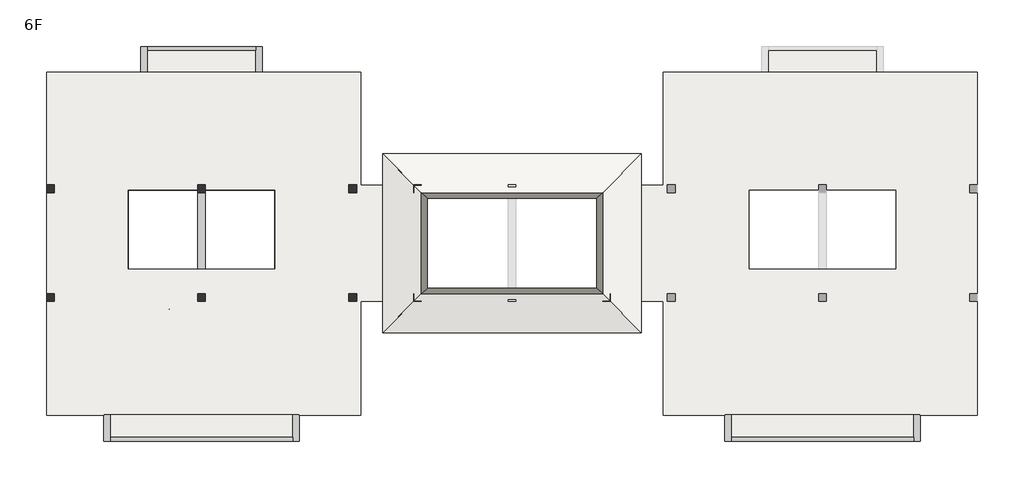
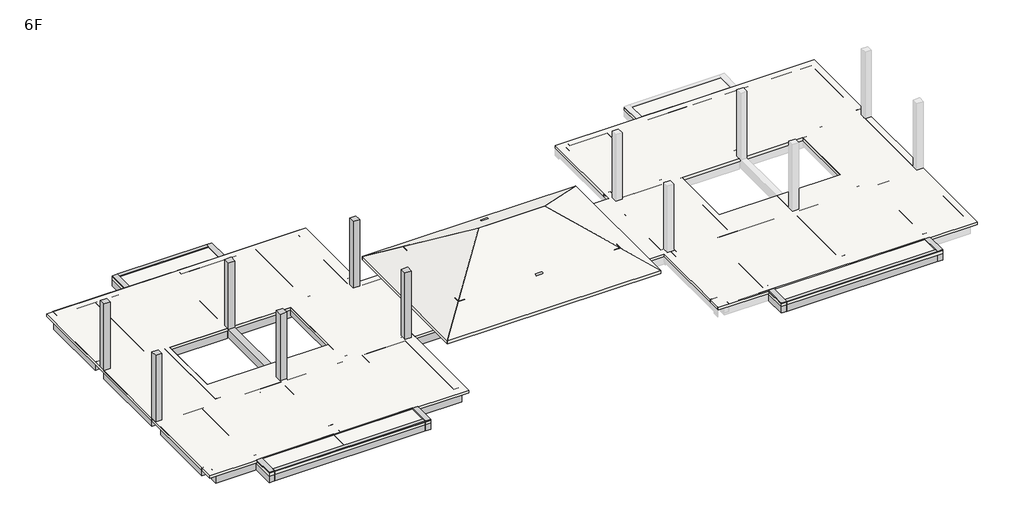
# One storey, part 1 of 2: 38 beams, 8 columns, 6 slabs.
"""IFC4 building model written with IfcOpenShell, lengths in millimetres."""

from ifc_helpers import new_model, si_unit, frame, origin, place, context, project, spatial, polyline, outline, extrude, faceted_brep, element, save

model = new_model("IFC4")

# Units and contexts
model_context = context("Model", 3, world=origin())
ifc_project = project(units=[si_unit("LENGTHUNIT", "METRE", prefix="MILLI")], contexts=[model_context])

# Site, building, storey
site = spatial("IfcSite", under=ifc_project)
building = spatial("IfcBuilding", under=site)
storey = spatial("IfcBuildingStorey", under=building, Name="6F", Elevation=17230.0)

# Beams
placement = place(None, origin())
element("IfcBeam", 1, ObjectType="M_Concrete-Rectangular Beam : 150x500", at=placement, inside=storey, context=model_context, shape_type="SweptSolid", body=[
    extrude(outline(polyline([(2320.0000398, -1149.9999999), (2320.0000398, -999.9999999), (9380.0000399, -999.9999999), (9380.0000399, -1149.9999999), (2320.0000398, -1149.9999999)])), frame((0.0, 0.0, 16730.0), z_axis=(0.0, 0.0, 1.0), x_axis=(1.0, 0.0, 0.0)), (0.0, 0.0, 1.0), 500.0),
])
element("IfcBeam", 2, ObjectType="M_Concrete-Rectangular Beam : 150x500", at=placement, inside=storey, context=model_context, shape_type="SweptSolid", body=[
    extrude(outline(polyline([(26320.012858, -1149.9999998), (26320.012858, -999.9999998), (33380.0128581, -999.9999998), (33380.0128581, -1149.9999998), (26320.012858, -1149.9999998)])), frame((0.0, 0.0, 16730.0), z_axis=(0.0, 0.0, 1.0), x_axis=(1.0, 0.0, 0.0)), (0.0, 0.0, 1.0), 500.0),
])
element("IfcBeam", 3, ObjectType="M_Concrete-Rectangular Beam : 150x500", at=placement, inside=storey, context=model_context, shape_type="SweptSolid", body=[
    extrude(outline(polyline([(7940.0998269, 14100.0000002), (7940.0998269, 13950.0000002), (3759.9001745, 13950.0000002), (3759.9001745, 14100.0000002), (7940.0998269, 14100.0000002)])), frame((0.0, 0.0, 16730.0), z_axis=(0.0, 0.0, 1.0), x_axis=(1.0, 0.0, 0.0)), (0.0, 0.0, 1.0), 500.0),
])
element("IfcBeam", 4, ObjectType="M_Concrete-Rectangular Beam : 250x400", at=placement, inside=storey, context=model_context, shape_type="Brep", body=[
    faceted_brep([(8930.0, 8549.9999993, 17230.0), (8680.0, 8549.9999993, 17230.0), (8680.0, 4449.9999998, 17230.0), (8930.0, 4449.9999998, 17230.0), (8680.0, 8549.9999993, 17088.8582236), (8680.0, 8549.9999993, 16830.0), (8680.0, 4449.9999998, 16830.0), (8930.0, 8549.9999993, 16830.0), (8930.0, 4449.9999998, 16830.0)], [[[0, 1, 2, 3]], [[1, 4, 5, 6, 2]], [[5, 7, 8, 6]], [[7, 0, 3, 8]], [[1, 0, 7, 5, 4]], [[3, 2, 6, 8]]]),
])
element("IfcBeam", 5, ObjectType="M_Concrete-Rectangular Beam : 250x400", at=placement, inside=storey, context=model_context, shape_type="SweptSolid", body=[
    extrude(outline(polyline([(14050.0174941, 8449.9999993), (14300.0174941, 8449.9999993), (14300.0174941, 4549.9999902), (14050.0174941, 4549.9999902), (14050.0174941, 8449.9999993)])), frame((0.0, 0.0, 16830.0), z_axis=(0.0, 0.0, 1.0), x_axis=(1.0, 0.0, 0.0)), (0.0, 0.0, 1.0), 400.0),
])
element("IfcBeam", 6, ObjectType="M_Concrete-Rectangular Beam : 250x400", at=placement, inside=storey, context=model_context, shape_type="Brep", body=[
    faceted_brep([(3020.0, 8549.9999993, 17230.0), (2770.0, 8549.9999993, 17230.0), (2770.0, 4449.9999998, 17230.0), (3020.0, 4449.9999998, 17230.0), (3020.0, 8549.9999993, 16830.0), (3020.0, 8549.9999993, 17088.8582245), (3020.0, 4449.9999998, 16830.0), (2770.0, 8549.9999993, 16830.0), (2770.0, 4449.9999998, 16830.0)], [[[0, 1, 2, 3]], [[4, 5, 0, 3, 6]], [[7, 4, 6, 8]], [[1, 7, 8, 2]], [[1, 0, 5, 4, 7]], [[3, 2, 8, 6]]]),
])
element("IfcBeam", 7, ObjectType="M_Concrete-Rectangular Beam : 250x400", at=placement, inside=storey, context=model_context, shape_type="SweptSolid", body=[
    extrude(outline(polyline([(1965.3131971, 12800.0000001), (2215.3131971, 12800.0000001), (2215.3131971, 8849.9999993), (1965.3131971, 8849.9999993), (1965.3131971, 12800.0000001)])), frame((0.0, 0.0, 16830.0), z_axis=(0.0, 0.0, 1.0), x_axis=(1.0, 0.0, 0.0)), (0.0, 0.0, 1.0), 400.0),
])
element("IfcBeam", 8, ObjectType="M_Concrete-Rectangular Beam : 250x400", at=placement, inside=storey, context=model_context, shape_type="SweptSolid", body=[
    extrude(outline(polyline([(1965.3131971, 4149.9999998), (2215.3131971, 4149.9999998), (2215.3131971, 199.9999993), (1965.3131971, 199.9999993), (1965.3131971, 4149.9999998)])), frame((0.0, 0.0, 16830.0), z_axis=(0.0, 0.0, 1.0), x_axis=(1.0, 0.0, 0.0)), (0.0, 0.0, 1.0), 400.0),
])
element("IfcBeam", 9, ObjectType="M_Concrete-Rectangular Beam : 250x400", at=placement, inside=storey, context=model_context, shape_type="SweptSolid", body=[
    extrude(outline(polyline([(9485.2332382, 12800.0000001), (9735.2332382, 12800.0000001), (9735.2332382, 8849.9999993), (9485.2332382, 8849.9999993), (9485.2332382, 12800.0000001)])), frame((0.0, 0.0, 16830.0), z_axis=(0.0, 0.0, 1.0), x_axis=(1.0, 0.0, 0.0)), (0.0, 0.0, 1.0), 400.0),
])
element("IfcBeam", 10, ObjectType="M_Concrete-Rectangular Beam : 250x400", at=placement, inside=storey, context=model_context, shape_type="SweptSolid", body=[
    extrude(outline(polyline([(9485.2332382, 4149.9999998), (9735.2332382, 4149.9999998), (9735.2332382, 199.9999993), (9485.2332382, 199.9999993), (9485.2332382, 4149.9999998)])), frame((0.0, 0.0, 16830.0), z_axis=(0.0, 0.0, 1.0), x_axis=(1.0, 0.0, 0.0)), (0.0, 0.0, 1.0), 400.0),
])
element("IfcBeam", 11, ObjectType="M_Concrete-Rectangular Beam : 250x400", at=placement, inside=storey, context=model_context, shape_type="SweptSolid", body=[
    extrude(outline(polyline([(17780.0, 14075.0174936), (17780.0, 14325.0174936), (18180.0, 14325.0174936), (18180.0, 14191.5713263), (18102.3013889, 14075.0174936), (17780.0, 14075.0174936)])), frame((0.0, 4550.0000005, 0.0), z_axis=(0.0, 1.0, 0.0), x_axis=(0.0, 0.0, 1.0)), (0.0, 0.0, 1.0), 3899.9999997),
])
element("IfcBeam", 12, ObjectType="M_Concrete-Rectangular Beam : 250x500", at=placement, inside=storey, context=model_context, shape_type="Brep", body=[
    faceted_brep([(3509.9001745, 13101.5853605, 17230.0), (3509.9001745, 13101.5853605, 16730.0), (3759.9001745, 13101.5853605, 16730.0), (3759.9001745, 13101.5853605, 17230.0), (3759.9001745, 13950.0000002, 17230.0), (3759.9001745, 14100.0000002, 17230.0), (3509.9001745, 14100.0000002, 17230.0), (3759.9001745, 13950.0000002, 16730.0), (3759.9001745, 14100.0000002, 16730.0), (3509.9001745, 14100.0000002, 16730.0)], [[[0, 1, 2, 3]], [[0, 3, 4, 5, 6]], [[3, 2, 7, 8, 5, 4]], [[2, 1, 9, 8, 7]], [[1, 0, 6, 9]], [[6, 5, 8, 9]]]),
])
element("IfcBeam", 13, ObjectType="M_Concrete-Rectangular Beam : 250x500", at=placement, inside=storey, context=model_context, shape_type="Brep", body=[
    faceted_brep([(2070.0000398, -1149.9999999, 17230.0), (2320.0000398, -1149.9999999, 17230.0), (2320.0000398, -999.9999999, 17230.0), (2320.0000398, -100.0000007, 17230.0), (2070.0000398, -100.0000007, 17230.0), (2320.0000398, -1149.9999999, 16730.0), (2320.0000398, -999.9999999, 16730.0), (2320.0000398, -100.0000007, 16730.0), (2070.0000398, -1149.9999999, 16730.0), (2070.0000398, -100.0000007, 16730.0)], [[[0, 1, 2, 3, 4]], [[1, 5, 6, 7, 3, 2]], [[5, 8, 9, 7, 6]], [[8, 0, 4, 9]], [[4, 3, 7, 9]], [[1, 0, 8, 5]]]),
])
element("IfcBeam", 14, ObjectType="M_Concrete-Rectangular Beam : 250x500", at=placement, inside=storey, context=model_context, shape_type="Brep", body=[
    faceted_brep([(9380.0000399, -1149.9999999, 17230.0), (9630.0000399, -1149.9999999, 17230.0), (9630.0000399, -100.0000007, 17230.0), (9380.0000399, -100.0000007, 17230.0), (9380.0000399, -999.9999999, 17230.0), (9380.0000399, -1149.9999999, 16730.0), (9380.0000399, -100.0000007, 16730.0), (9380.0000399, -999.9999999, 16730.0), (9630.0000399, -1149.9999999, 16730.0), (9630.0000399, -100.0000007, 16730.0)], [[[0, 1, 2, 3, 4]], [[5, 0, 4, 3, 6, 7]], [[8, 5, 7, 6, 9]], [[1, 8, 9, 2]], [[1, 0, 5, 8]], [[3, 2, 9, 6]]]),
])
element("IfcBeam", 15, ObjectType="M_Concrete-Rectangular Beam : 250x500", at=placement, inside=storey, context=model_context, shape_type="Brep", body=[
    faceted_brep([(26070.012858, -1149.9999998, 17230.0), (26320.012858, -1149.9999998, 17230.0), (26320.012858, -999.9999998, 17230.0), (26320.012858, -100.0000013, 17230.0), (26070.012858, -100.0000013, 17230.0), (26320.012858, -1149.9999998, 16730.0), (26320.012858, -999.9999998, 16730.0), (26320.012858, -100.0000013, 16730.0), (26070.012858, -1149.9999998, 16730.0), (26070.012858, -100.0000013, 16730.0)], [[[0, 1, 2, 3, 4]], [[1, 5, 6, 7, 3, 2]], [[5, 8, 9, 7, 6]], [[8, 0, 4, 9]], [[1, 0, 8, 5]], [[4, 3, 7, 9]]]),
])
element("IfcBeam", 16, ObjectType="M_Concrete-Rectangular Beam : 250x500", at=placement, inside=storey, context=model_context, shape_type="Brep", body=[
    faceted_brep([(33380.0128581, -1149.9999998, 17230.0), (33630.0128581, -1149.9999998, 17230.0), (33630.0128581, -100.0000013, 17230.0), (33380.0128581, -100.0000013, 17230.0), (33380.0128581, -999.9999998, 17230.0), (33380.0128581, -1149.9999998, 16730.0), (33380.0128581, -100.0000013, 16730.0), (33380.0128581, -999.9999998, 16730.0), (33630.0128581, -1149.9999998, 16730.0), (33630.0128581, -100.0000013, 16730.0)], [[[0, 1, 2, 3, 4]], [[5, 0, 4, 3, 6, 7]], [[8, 5, 7, 6, 9]], [[1, 8, 9, 2]], [[1, 0, 5, 8]], [[3, 2, 9, 6]]]),
])
element("IfcBeam", 17, ObjectType="M_Concrete-Rectangular Beam : 250x500", at=placement, inside=storey, context=model_context, shape_type="Brep", body=[
    faceted_brep([(8190.0998269, 14100.0000002, 17230.0), (7940.0998269, 14100.0000002, 17230.0), (7940.0998269, 13950.0000002, 17230.0), (7940.0998269, 13100.0000001, 17230.0), (8190.0998269, 13100.0000001, 17230.0), (8190.0998269, 14100.0000002, 16730.0), (8190.0998269, 13100.0000001, 16730.0), (7940.0998269, 14100.0000002, 16730.0), (7940.0998269, 13100.0000001, 16730.0), (7940.0998269, 13950.0000002, 16730.0)], [[[0, 1, 2, 3, 4]], [[5, 0, 4, 6]], [[7, 5, 6, 8, 9]], [[1, 7, 9, 8, 3, 2]], [[1, 0, 5, 7]], [[4, 3, 8, 6]]]),
])
element("IfcBeam", 18, ObjectType="M_Concrete-Rectangular Beam : 300x400", at=placement, inside=storey, context=model_context, shape_type="SweptSolid", body=[
    extrude(outline(polyline([(165.0, 9150.0000002), (-135.0, 9150.0000002), (-135.0, 12500.0000005), (165.0, 12500.0000005), (165.0, 9150.0000002)])), frame((0.0, 0.0, 16830.0), z_axis=(0.0, 0.0, 1.0), x_axis=(1.0, 0.0, 0.0)), (0.0, 0.0, 1.0), 400.0),
])
element("IfcBeam", 19, ObjectType="M_Concrete-Rectangular Beam : 300x400", at=placement, inside=storey, context=model_context, shape_type="SweptSolid", body=[
    extrude(outline(polyline([(165.0, 4550.0000002), (-135.0, 4550.0000002), (-135.0, 8450.0000002), (165.0, 8450.0000002), (165.0, 4550.0000002)])), frame((0.0, 0.0, 16830.0), z_axis=(0.0, 0.0, 1.0), x_axis=(1.0, 0.0, 0.0)), (0.0, 0.0, 1.0), 400.0),
])
element("IfcBeam", 20, ObjectType="M_Concrete-Rectangular Beam : 300x400", at=placement, inside=storey, context=model_context, shape_type="SweptSolid", body=[
    extrude(outline(polyline([(165.0, 500.0), (-135.0, 500.0), (-135.0, 3850.0000002), (165.0, 3850.0000002), (165.0, 500.0)])), frame((0.0, 0.0, 16830.0), z_axis=(0.0, 0.0, 1.0), x_axis=(1.0, 0.0, 0.0)), (0.0, 0.0, 1.0), 400.0),
])
element("IfcBeam", 21, ObjectType="M_Concrete-Rectangular Beam : 300x400", at=placement, inside=storey, context=model_context, shape_type="SweptSolid", body=[
    extrude(outline(polyline([(6000.0, 4550.0000002), (5700.0, 4550.0000002), (5700.0, 8450.0000002), (6000.0, 8450.0000002), (6000.0, 4550.0000002)])), frame((0.0, 0.0, 16830.0), z_axis=(0.0, 0.0, 1.0), x_axis=(1.0, 0.0, 0.0)), (0.0, 0.0, 1.0), 400.0),
])
element("IfcBeam", 22, ObjectType="M_Concrete-Rectangular Beam : 300x400", at=placement, inside=storey, context=model_context, shape_type="SweptSolid", body=[
    extrude(outline(polyline([(6000.0000007, 500.0), (5700.0000007, 500.0), (5700.0000007, 3850.0000002), (6000.0000007, 3850.0000002), (6000.0000007, 500.0)])), frame((0.0, 0.0, 16830.0), z_axis=(0.0, 0.0, 1.0), x_axis=(1.0, 0.0, 0.0)), (0.0, 0.0, 1.0), 400.0),
])
element("IfcBeam", 23, ObjectType="M_Concrete-Rectangular Beam : 300x400", at=placement, inside=storey, context=model_context, shape_type="SweptSolid", body=[
    extrude(outline(polyline([(6000.0000007, 9150.0000002), (5700.0000007, 9150.0000002), (5700.0000007, 12500.0000005), (6000.0000007, 12500.0000005), (6000.0000007, 9150.0000002)])), frame((0.0, 0.0, 16830.0), z_axis=(0.0, 0.0, 1.0), x_axis=(1.0, 0.0, 0.0)), (0.0, 0.0, 1.0), 400.0),
])
element("IfcBeam", 24, ObjectType="M_Concrete-Rectangular Beam : 300x400", at=placement, inside=storey, context=model_context, shape_type="Brep", body=[
    faceted_brep([(6000.0000007, -100.0, 17180.0), (5700.0000007, -100.0000007, 17180.0), (5700.0000007, -999.9999999, 17180.0), (6000.0000007, -999.9999999, 17180.0), (6000.0000007, -999.9999999, 16780.0), (6000.0000007, -100.0, 16780.0), (5700.0000007, -100.0000007, 16780.0), (5700.0000007, -999.9999999, 16780.0)], [[[0, 1, 2, 3]], [[3, 4, 5, 0]], [[6, 5, 4, 7]], [[1, 6, 7, 2]], [[0, 5, 6, 1]], [[3, 2, 7, 4]]]),
])
element("IfcBeam", 25, ObjectType="M_Concrete-Rectangular Beam : 300x400", at=placement, inside=storey, context=model_context, shape_type="Brep", body=[
    faceted_brep([(30000.0064292, -100.0, 17180.0), (29700.0064292, -100.0000013, 17180.0), (29700.0064292, -999.9999998, 17180.0), (30000.0064292, -999.9999998, 17180.0), (30000.0064292, -999.9999998, 16780.0), (30000.0064292, -100.0, 16780.0), (29700.0064292, -100.0000013, 16780.0), (29700.0064292, -999.9999998, 16780.0)], [[[0, 1, 2, 3]], [[3, 4, 5, 0]], [[6, 5, 4, 7]], [[1, 6, 7, 2]], [[0, 5, 6, 1]], [[3, 2, 7, 4]]]),
])
element("IfcBeam", 26, ObjectType="M_Concrete-Rectangular Beam : 300x500", at=placement, inside=storey, context=model_context, shape_type="Brep", body=[
    faceted_brep([(5700.0000007, 12800.0000001, 17230.0), (5700.0000007, 13100.0000001, 17230.0), (165.0, 13100.0000001, 17230.0), (165.0, 12800.0000001, 17230.0), (1965.3131971, 12800.0000001, 17230.0), (2215.3131971, 12800.0000001, 17230.0), (5700.0000007, 12800.0000001, 16730.0), (165.0, 12800.0000001, 16730.0), (5700.0000007, 13100.0000001, 16730.0), (165.0, 13100.0000001, 16730.0)], [[[0, 1, 2, 3, 4, 5]], [[6, 0, 5, 4, 3, 7]], [[8, 6, 7, 9]], [[1, 8, 9, 2]], [[1, 0, 6, 8]], [[3, 2, 9, 7]]]),
])
element("IfcBeam", 27, ObjectType="M_Concrete-Rectangular Beam : 300x500", at=placement, inside=storey, context=model_context, shape_type="Brep", body=[
    faceted_brep([(164.9649925, 8849.9999993, 17230.0), (164.9649925, 8549.9999993, 17230.0), (2770.0, 8549.9999993, 17230.0), (3020.0, 8549.9999993, 17230.0), (5699.9649933, 8549.9999993, 17230.0), (5699.9649933, 8849.9999993, 17230.0), (2215.3131971, 8849.9999993, 17230.0), (1965.3131971, 8849.9999993, 17230.0), (164.9649925, 8549.9999993, 16730.0), (5699.9649933, 8549.9999993, 16730.0), (164.9649925, 8849.9999993, 16730.0), (5699.9649933, 8849.9999993, 16730.0)], [[[0, 1, 2, 3, 4, 5, 6, 7]], [[1, 8, 9, 4, 3, 2]], [[8, 10, 11, 9]], [[10, 0, 7, 6, 5, 11]], [[1, 0, 10, 8]], [[5, 4, 9, 11]]]),
])
element("IfcBeam", 28, ObjectType="M_Concrete-Rectangular Beam : 300x500", at=placement, inside=storey, context=model_context, shape_type="Brep", body=[
    faceted_brep([(165.0, 4449.9999998, 17230.0), (165.0, 4149.9999998, 17230.0), (1965.3131971, 4149.9999998, 17230.0), (2215.3131971, 4149.9999998, 17230.0), (5700.0000007, 4149.9999998, 17230.0), (5700.0000007, 4449.9999998, 17230.0), (3020.0, 4449.9999998, 17230.0), (2770.0, 4449.9999998, 17230.0), (165.0, 4149.9999998, 16730.0), (5700.0000007, 4149.9999998, 16730.0), (165.0, 4449.9999998, 16730.0), (5700.0000007, 4449.9999998, 16730.0)], [[[0, 1, 2, 3, 4, 5, 6, 7]], [[1, 8, 9, 4, 3, 2]], [[8, 10, 11, 9]], [[10, 0, 7, 6, 5, 11]], [[1, 0, 10, 8]], [[5, 4, 9, 11]]]),
])
element("IfcBeam", 29, ObjectType="M_Concrete-Rectangular Beam : 300x500", at=placement, inside=storey, context=model_context, shape_type="Brep", body=[
    faceted_brep([(165.0, 199.9999993, 17230.0), (165.0, -100.0000007, 17230.0), (2070.0000398, -100.0000007, 17230.0), (2320.0000398, -100.0000007, 17230.0), (5700.0000007, -100.0000007, 17230.0), (5700.0000007, 199.9999993, 17230.0), (2215.3131971, 199.9999993, 17230.0), (1965.3131971, 199.9999993, 17230.0), (165.0, -100.0000007, 16730.0), (2070.0000398, -100.0000007, 16730.0), (2320.0000398, -100.0000007, 16730.0), (5700.0000007, -100.0000007, 16730.0), (165.0, 199.9999993, 16730.0), (5700.0000007, 199.9999993, 16730.0)], [[[0, 1, 2, 3, 4, 5, 6, 7]], [[1, 8, 9, 10, 11, 4, 3, 2]], [[8, 12, 13, 11, 10, 9]], [[12, 0, 7, 6, 5, 13]], [[1, 0, 12, 8]], [[5, 4, 11, 13]]]),
])
element("IfcBeam", 30, ObjectType="M_Concrete-Rectangular Beam : 300x500", at=placement, inside=storey, context=model_context, shape_type="Brep", body=[
    faceted_brep([(6000.0000007, 13100.0000001, 17230.0), (6000.0000007, 12800.0000001, 17230.0), (9485.2332382, 12800.0000001, 17230.0), (9735.2332382, 12800.0000001, 17230.0), (11500.0174948, 12800.0000001, 17230.0), (11700.0000034, 12800.0000001, 17230.0), (11700.0000034, 13100.0000001, 17230.0), (8190.0998269, 13100.0000001, 17230.0), (7940.0998269, 13100.0000001, 17230.0), (6000.0000007, 12800.0000001, 16730.0), (11700.0000034, 12800.0000001, 16730.0), (11700.0000034, 12800.0000001, 16830.0), (6000.0000007, 13100.0000001, 16730.0), (7940.0998269, 13100.0000001, 16730.0), (8190.0998269, 13100.0000001, 16730.0), (11700.0000034, 13100.0000001, 16730.0)], [[[0, 1, 2, 3, 4, 5, 6, 7, 8]], [[1, 9, 10, 11, 5, 4, 3, 2]], [[9, 12, 13, 14, 15, 10]], [[12, 0, 8, 7, 6, 15, 14, 13]], [[1, 0, 12, 9]], [[6, 5, 11, 10, 15]]]),
])
element("IfcBeam", 31, ObjectType="M_Concrete-Rectangular Beam : 300x500", at=placement, inside=storey, context=model_context, shape_type="Brep", body=[
    faceted_brep([(5999.9649933, 8849.9999993, 17230.0), (5999.9649933, 8549.9999993, 17230.0), (8680.0, 8549.9999993, 17230.0), (8930.0, 8549.9999993, 17230.0), (11500.0174941, 8549.9999993, 17230.0), (11699.964996, 8549.9999993, 17230.0), (11699.964996, 8849.9999993, 17230.0), (11500.0174948, 8849.9999993, 17230.0), (9735.2332382, 8849.9999993, 17230.0), (9485.2332382, 8849.9999993, 17230.0), (5999.9649933, 8549.9999993, 16730.0), (11500.0174941, 8549.9999993, 16730.0), (11699.964996, 8549.9999993, 16730.0), (11699.964996, 8549.9999993, 16830.0), (5999.9649933, 8849.9999993, 16730.0), (11699.964996, 8849.9999993, 16730.0), (11699.964996, 8849.9999993, 16830.0)], [[[0, 1, 2, 3, 4, 5, 6, 7, 8, 9]], [[1, 10, 11, 12, 13, 5, 4, 3, 2]], [[10, 14, 15, 12, 11]], [[14, 0, 9, 8, 7, 6, 16, 15]], [[1, 0, 14, 10]], [[6, 5, 13, 12, 15, 16]]]),
])
element("IfcBeam", 32, ObjectType="M_Concrete-Rectangular Beam : 300x500", at=placement, inside=storey, context=model_context, shape_type="Brep", body=[
    faceted_brep([(6000.0000007, 4449.9999998, 17230.0), (6000.0000007, 4149.9999998, 17230.0), (9485.2332382, 4149.9999998, 17230.0), (9735.2332382, 4149.9999998, 17230.0), (11500.0174948, 4149.9999998, 17230.0), (11700.0000034, 4149.9999998, 17230.0), (11700.0000034, 4449.9999998, 17230.0), (11500.0174941, 4449.9999998, 17230.0), (8930.0, 4449.9999998, 17230.0), (8680.0, 4449.9999998, 17230.0), (6000.0000007, 4149.9999998, 16730.0), (11700.0000034, 4149.9999998, 16730.0), (11700.0000034, 4149.9999998, 16830.0), (6000.0000007, 4449.9999998, 16730.0), (11500.0174948, 4449.9999998, 16730.0), (11700.0000034, 4449.9999998, 16730.0), (11700.0000034, 4449.9999998, 16830.0)], [[[0, 1, 2, 3, 4, 5, 6, 7, 8, 9]], [[1, 10, 11, 12, 5, 4, 3, 2]], [[10, 13, 14, 15, 11]], [[13, 0, 9, 8, 7, 6, 16, 15, 14]], [[1, 0, 13, 10]], [[6, 5, 12, 11, 15, 16]]]),
])
element("IfcBeam", 33, ObjectType="M_Concrete-Rectangular Beam : 300x500", at=placement, inside=storey, context=model_context, shape_type="Brep", body=[
    faceted_brep([(6000.0000007, 199.9999993, 17230.0), (6000.0000007, -100.0000007, 17230.0), (9380.0000399, -100.0000007, 17230.0), (9630.0000399, -100.0000007, 17230.0), (11700.0000034, -100.0000007, 17230.0), (11700.0000034, 199.9999993, 17230.0), (11500.0174948, 199.9999993, 17230.0), (9735.2332382, 199.9999993, 17230.0), (9485.2332382, 199.9999993, 17230.0), (6000.0000007, -100.0000007, 16730.0), (9380.0000399, -100.0000007, 16730.0), (9630.0000399, -100.0000007, 16730.0), (11700.0000034, -100.0000007, 16730.0), (6000.0000007, 199.9999993, 16730.0), (11700.0000034, 199.9999993, 16730.0), (11700.0000034, 199.9999993, 16830.0)], [[[0, 1, 2, 3, 4, 5, 6, 7, 8]], [[1, 9, 10, 11, 12, 4, 3, 2]], [[9, 13, 14, 12, 11, 10]], [[13, 0, 8, 7, 6, 5, 15, 14]], [[1, 0, 13, 9]], [[5, 4, 12, 14, 15]]]),
])
element("IfcBeam", 34, ObjectType="M_Concrete-Rectangular Beam : 300x500", at=placement, inside=storey, context=model_context, shape_type="Brep", body=[
    faceted_brep([(17699.9649983, 8449.9999993, 17230.0), (17699.9649983, 8749.9999993, 17230.0), (12000.0174941, 8749.9999993, 17230.0), (12000.0174941, 8549.9999993, 17230.0), (12000.0174941, 8449.9999993, 17230.0), (14050.0174941, 8449.9999993, 17230.0), (14300.0174941, 8449.9999993, 17230.0), (17699.9649983, 8449.9999993, 16730.0), (11999.964996, 8449.9999993, 16730.0), (17699.9649983, 8749.9999993, 16730.0), (11999.964996, 8549.9999993, 16730.0), (11999.964996, 8749.9999993, 16730.0)], [[[0, 1, 2, 3, 4, 5, 6]], [[7, 0, 6, 5, 4, 8]], [[9, 7, 8, 10, 11]], [[1, 9, 11, 2]], [[2, 11, 10, 8, 4, 3]], [[1, 0, 7, 9]]]),
    faceted_brep([(11500.0174941, 8449.9999993, 16830.0), (11699.964996, 8449.9999993, 16830.0), (11699.964996, 8549.9999993, 16830.0), (11500.0174941, 8549.9999993, 16830.0), (11500.0174941, 8449.9999993, 16730.0), (11500.0174941, 8549.9999993, 16730.0), (11699.964996, 8449.9999993, 16730.0), (11699.964996, 8549.9999993, 16730.0)], [[[0, 1, 2, 3]], [[4, 0, 3, 5]], [[1, 6, 7, 2]], [[0, 4, 6, 1]], [[6, 4, 5, 7]], [[3, 2, 7, 5]]]),
])
element("IfcBeam", 35, ObjectType="M_Concrete-Rectangular Beam : 300x500", at=placement, inside=storey, context=model_context, shape_type="Brep", body=[
    faceted_brep([(17700.0000058, 4249.9999902, 17230.0), (17700.0000058, 4549.9999902, 17230.0), (14300.0174941, 4549.9999902, 17230.0), (14050.0174941, 4549.9999902, 17230.0), (12000.0174941, 4549.9999902, 17230.0), (12000.0174941, 4449.9999998, 17230.0), (12000.0174941, 4249.9999902, 17230.0), (17700.0000058, 4249.9999902, 16730.0), (12000.0000034, 4249.9999902, 16730.0), (17700.0000058, 4549.9999902, 16730.0), (12000.0000034, 4449.9999998, 16730.0), (12000.0000034, 4549.9999902, 16730.0)], [[[0, 1, 2, 3, 4, 5, 6]], [[7, 0, 6, 8]], [[9, 7, 8, 10, 11]], [[1, 9, 11, 4, 3, 2]], [[4, 11, 10, 8, 6, 5]], [[1, 0, 7, 9]]]),
    faceted_brep([(11700.0000034, 4549.9999902, 16830.0), (11500.0174948, 4549.9999902, 16830.0), (11500.0174948, 4449.9999998, 16830.0), (11700.0000034, 4449.9999998, 16830.0), (11500.0174948, 4549.9999902, 16730.0), (11500.0174948, 4449.9999998, 16730.0), (11700.0000034, 4549.9999902, 16730.0), (11700.0000034, 4449.9999998, 16730.0)], [[[0, 1, 2, 3]], [[1, 4, 5, 2]], [[6, 0, 3, 7]], [[4, 6, 7, 5]], [[4, 1, 0, 6]], [[3, 2, 5, 7]]]),
])
element("IfcBeam", 36, ObjectType="M_Concrete-Rectangular Beam : 500x400", at=placement, inside=storey, context=model_context, shape_type="Brep", body=[
    faceted_brep([(11700.0000034, 4449.9999998, 17230.0), (11700.0000034, 4550.0000002, 17230.0), (12000.0174941, 4550.0000002, 17230.0), (12000.0174941, 8450.0000002, 17230.0), (11699.964996, 8450.0000002, 17230.0), (11699.964996, 8549.9999993, 17230.0), (11500.0174941, 8549.9999993, 17230.0), (11500.0174941, 4449.9999998, 17230.0), (12000.0174941, 4550.0000002, 16830.0), (12000.0174941, 8450.0000002, 16830.0), (11700.0000034, 4550.0000002, 16830.0), (11700.0000034, 4449.9999998, 16830.0), (11500.0174941, 4449.9999998, 16830.0), (11500.0174941, 8449.9999993, 16830.0), (11500.0174941, 8549.9999993, 16830.0), (11699.964996, 8549.9999993, 16830.0), (11699.964996, 8450.0000002, 16830.0)], [[[0, 1, 2, 3, 4, 5, 6, 7]], [[2, 8, 9, 3]], [[10, 11, 12, 13, 14, 15, 16, 9, 8]], [[6, 14, 13, 12, 7]], [[14, 6, 5, 15]], [[7, 12, 11, 0]], [[10, 1, 0, 11]], [[1, 10, 8, 2]], [[16, 4, 3, 9]], [[4, 16, 15, 5]]]),
])
element("IfcBeam", 37, ObjectType="M_Concrete-Rectangular Beam : 500x400", at=placement, inside=storey, context=model_context, shape_type="SweptSolid", body=[
    extrude(outline(polyline([(11700.0000034, 500.0), (11700.0000034, 199.9999993), (11500.0174948, 199.9999993), (11500.0174948, 4149.9999998), (11700.0000034, 4149.9999998), (11700.0000034, 3850.0000002), (12000.0174948, 3850.0000002), (12000.0174948, 500.0), (11700.0000034, 500.0)])), frame((0.0, 0.0, 16830.0), z_axis=(0.0, 0.0, 1.0), x_axis=(1.0, 0.0, 0.0)), (0.0, 0.0, 1.0), 400.0),
])
element("IfcBeam", 38, ObjectType="M_Concrete-Rectangular Beam : 500x400", at=placement, inside=storey, context=model_context, shape_type="SweptSolid", body=[
    extrude(outline(polyline([(11699.964996, 9150.0000002), (11699.964996, 8849.9999993), (11500.0174948, 8849.9999993), (11500.0174948, 12800.0000001), (11700.0000034, 12800.0000001), (11700.0000034, 12500.0000005), (12000.0174948, 12500.0000005), (12000.0174948, 9150.0000002), (11699.964996, 9150.0000002)])), frame((0.0, 0.0, 16830.0), z_axis=(0.0, 0.0, 1.0), x_axis=(1.0, 0.0, 0.0)), (0.0, 0.0, 1.0), 400.0),
])

# Columns
element("IfcColumn", 39, ObjectType="M_Concrete-Rectangular-Column : 300x300", at=placement, inside=storey, context=model_context, shape_type="SweptSolid", body=[
    extrude(outline(polyline([(164.9649925, 4550.0000005), (164.9649925, 4250.0000005), (-135.0350075, 4250.0000005), (-135.0350075, 4550.0000005), (164.9649925, 4550.0000005)])), frame((0.0, 0.0, 17230.0), z_axis=(0.0, 0.0, 1.0), x_axis=(1.0, 0.0, 0.0)), (0.0, 0.0, 1.0), 3300.0),
])
element("IfcColumn", 40, ObjectType="M_Concrete-Rectangular-Column : 300x300", at=placement, inside=storey, context=model_context, shape_type="SweptSolid", body=[
    extrude(outline(polyline([(164.9649925, 8750.0000002), (164.9649925, 8450.0000002), (-135.0350075, 8450.0000002), (-135.0350075, 8750.0000002), (164.9649925, 8750.0000002)])), frame((0.0, 0.0, 17230.0), z_axis=(0.0, 0.0, 1.0), x_axis=(1.0, 0.0, 0.0)), (0.0, 0.0, 1.0), 3300.0),
])
element("IfcColumn", 41, ObjectType="M_Concrete-Rectangular-Column : 300x300", at=placement, inside=storey, context=model_context, shape_type="SweptSolid", body=[
    extrude(outline(polyline([(6000.0000012, 4550.0000005), (6000.0000012, 4250.0000005), (5700.0000012, 4250.0000005), (5700.0000012, 4550.0000005), (6000.0000012, 4550.0000005)])), frame((0.0, 0.0, 17230.0), z_axis=(0.0, 0.0, 1.0), x_axis=(1.0, 0.0, 0.0)), (0.0, 0.0, 1.0), 3300.0),
])
element("IfcColumn", 42, ObjectType="M_Concrete-Rectangular-Column : 300x300", at=placement, inside=storey, context=model_context, shape_type="SweptSolid", body=[
    extrude(outline(polyline([(6000.0000012, 8750.0000002), (6000.0000012, 8450.0000002), (5700.0000012, 8450.0000002), (5700.0000012, 8750.0000002), (6000.0000012, 8750.0000002)])), frame((0.0, 0.0, 17230.0), z_axis=(0.0, 0.0, 1.0), x_axis=(1.0, 0.0, 0.0)), (0.0, 0.0, 1.0), 3300.0),
])
element("IfcColumn", 43, ObjectType="M_Concrete-Rectangular-Column : 300x300", at=placement, inside=storey, context=model_context, shape_type="SweptSolid", body=[
    extrude(outline(polyline([(11850.000003, 4550.0000005), (11850.000003, 4250.0000005), (11550.000003, 4250.0000005), (11550.000003, 4550.0000005), (11850.000003, 4550.0000005)])), frame((0.0, 0.0, 17230.0), z_axis=(0.0, 0.0, 1.0), x_axis=(1.0, 0.0, 0.0)), (0.0, 0.0, 1.0), 3300.0),
])
element("IfcColumn", 44, ObjectType="M_Concrete-Rectangular-Column : 300x300", at=placement, inside=storey, context=model_context, shape_type="SweptSolid", body=[
    extrude(outline(polyline([(11850.000003, 8750.0000002), (11850.000003, 8450.0000002), (11550.000003, 8450.0000002), (11550.000003, 8750.0000002), (11850.000003, 8750.0000002)])), frame((0.0, 0.0, 17230.0), z_axis=(0.0, 0.0, 1.0), x_axis=(1.0, 0.0, 0.0)), (0.0, 0.0, 1.0), 3300.0),
])
element("IfcColumn", 45, ObjectType="M_Concrete-Rectangular-Column : 300x300", at=placement, inside=storey, context=model_context, shape_type="Brep", body=[
    faceted_brep([(14350.0174936, 4550.0000005, 17230.0), (14350.0174936, 4250.0000005, 17230.0), (14050.0174936, 4250.0000005, 17230.0), (14050.0174936, 4550.0000005, 17230.0), (14350.0174936, 4250.0000005, 18244.0536851), (14350.0174936, 4250.0000005, 18230.1951101), (14350.0174936, 4270.7873401, 18244.0536851), (14350.0174936, 4250.0000005, 18085.9719428), (14050.2926922, 4250.0000005, 18085.9719428), (14050.2926922, 4250.0000005, 18230.1951101), (14050.0174936, 4250.0000005, 18244.0536851), (14050.0174936, 4550.0000005, 18244.0536851), (14350.0174936, 4550.0000005, 18244.0536851), (14071.0805551, 4270.7873401, 18244.0536851), (14287.4153095, 4487.1166494, 18244.0536851), (14350.0174936, 4487.1166494, 18244.0536851)], [[[0, 1, 2, 3]], [[4, 5, 6]], [[2, 1, 7, 8, 9, 5, 4, 10]], [[3, 2, 10, 11]], [[0, 3, 11, 12]], [[10, 4, 6, 13, 14, 15, 12, 11]], [[14, 8, 7, 15]], [[9, 13, 6, 5]], [[8, 14, 13, 9]], [[1, 0, 12, 15, 7]]]),
])
element("IfcColumn", 46, ObjectType="M_Concrete-Rectangular-Column : 300x300", at=placement, inside=storey, context=model_context, shape_type="Brep", body=[
    faceted_brep([(14350.0174936, 8750.0000002, 17230.0), (14350.0174936, 8450.0000002, 17230.0), (14050.0174936, 8450.0000002, 17230.0), (14050.0174936, 8750.0000002, 17230.0), (14350.0174936, 8750.0000002, 18229.8452157), (14350.0174936, 8750.0000002, 18244.0536851), (14350.0174936, 8728.6878321, 18244.0536851), (14350.0174936, 8450.0000002, 18244.0536851), (14050.0174936, 8450.0000002, 18244.0536851), (14050.0174936, 8750.0000002, 18244.0536851), (14050.0174936, 8750.0000002, 18229.8452157), (14050.0174936, 8749.7503634, 18230.0116444), (14050.0174936, 8749.7503634, 18085.7884771), (14050.0174936, 8750.0000002, 18085.6220484), (14350.0174936, 8512.3585228, 18244.0536851), (14287.4153095, 8512.3585228, 18244.0536851), (14071.0805551, 8728.6878321, 18244.0536851), (14350.0174936, 8608.4366337, 18180.0), (14350.0174936, 8724.9999993, 18102.2891349), (14350.0174936, 8750.0000002, 18085.6220484)], [[[0, 1, 2, 3]], [[4, 5, 6]], [[2, 1, 7, 8]], [[3, 2, 8, 9, 10, 11, 12, 13]], [[9, 5, 4, 10]], [[8, 7, 14, 15, 16, 6, 5, 9]], [[12, 15, 14, 17, 18, 19, 13]], [[16, 11, 10, 4, 6]], [[15, 12, 11, 16]], [[1, 0, 19, 18, 17, 14, 7]], [[0, 3, 13, 19]]]),
])

# Slabs
element("IfcSlab", 47, ObjectType="120", at=placement, inside=storey, context=model_context, shape_type="Brep", body=[
    faceted_brep([(22849.8264693, 9949.7376449, 17285.7768327), (21649.7667691, 8749.6477389, 18085.8568952), (21499.8981776, 8599.7753751, 18185.7743176), (19400.0000833, 6499.8244256, 19585.7768327), (16300.0000636, 6499.8244256, 19585.7768327), (14287.4153095, 8512.3585228, 18244.0536851), (14050.0174936, 8749.7503634, 18085.7884771), (12850.0000076, 9949.7376449, 17285.7768327), (22849.8264693, 9949.7376449, 17430.0), (12850.0000076, 9949.7376449, 17430.0), (14050.0174936, 8749.7503634, 18230.0116444), (14071.0805551, 8728.6878321, 18244.0536851), (16300.0000636, 6499.8244256, 19730.0), (19400.0000833, 6499.8244256, 19730.0)], [[[0, 1, 2, 3, 4, 5, 6, 7]], [[8, 9, 10, 11, 12, 13]], [[0, 7, 9, 8]], [[3, 2, 1, 0, 8, 13]], [[4, 3, 13, 12]], [[7, 6, 5, 4, 12, 11, 10, 9]]]),
])
element("IfcSlab", 48, ObjectType="120", at=placement, inside=storey, context=model_context, shape_type="Brep", body=[
    faceted_brep([(22849.826469, 9949.7376446, 17285.7802013), (22849.826469, 3049.7375222, 17285.7802013), (19399.9132461, 6499.7375863, 19585.605611), (22849.826469, 9949.7376446, 17430.0), (19399.9132461, 6499.7375863, 19729.8254097), (22849.826469, 3049.7375222, 17430.0)], [[[0, 1, 2]], [[3, 4, 5]], [[1, 0, 3, 5]], [[2, 1, 5, 4]], [[0, 2, 4, 3]]]),
])
element("IfcSlab", 49, ObjectType="120", at=placement, inside=storey, context=model_context, shape_type="Brep", body=[
    faceted_brep([(22849.8264693, 3049.7375273, 17285.7768327), (12850.0000076, 3049.7375273, 17285.7768327), (14050.2926922, 4250.0000005, 18085.9719428), (14287.4153095, 4487.1166494, 18244.0536851), (16300.0000636, 6499.6507466, 19585.7768327), (19400.0000833, 6499.6507466, 19585.7768327), (22849.8264693, 3049.7375273, 17430.0), (19400.0000833, 6499.6507466, 19730.0), (16300.0000636, 6499.6507466, 19730.0), (14071.0805551, 4270.7873401, 18244.0536851), (14050.2926922, 4250.0000005, 18230.1951101), (12850.0000076, 3049.7375273, 17430.0)], [[[0, 1, 2, 3, 4, 5]], [[6, 7, 8, 9, 10, 11]], [[1, 0, 6, 11]], [[0, 5, 7, 6]], [[5, 4, 8, 7]], [[4, 3, 2, 1, 11, 10, 9, 8]]]),
])
element("IfcSlab", 50, ObjectType="120", at=placement, inside=storey, context=model_context, shape_type="Brep", body=[
    faceted_brep([(12850.1735425, 9949.7376446, 17285.7802013), (16300.0867655, 6499.7375863, 19585.605611), (12850.1735425, 3049.7375222, 17285.7802013), (12850.1735425, 9949.7376446, 17430.0), (12850.1735425, 3049.7375222, 17430.0), (16300.0867655, 6499.7375863, 19729.8254097)], [[[0, 1, 2]], [[3, 4, 5]], [[0, 2, 4, 3]], [[2, 1, 5, 4]], [[1, 0, 3, 5]]]),
])
element("IfcSlab", 51, ObjectType="130", at=placement, inside=storey, context=model_context, shape_type="SweptSolid", body=[
    extrude(outline(polyline([(5887.0630759, 13100.0000001), (12000.0174948, 13100.0000001), (12000.0174948, 8749.9999993), (23699.5160441, 8749.9999993), (23699.5160441, 13100.0000001), (29798.176913, 13100.0000001), (35835.035019, 13100.0000001), (35835.035019, -149.9999998), (33630.0128581, -149.9999998), (33630.0128581, -100.0000013), (26070.012858, -100.0000013), (26070.012858, -150.2407826), (23699.5160441, -150.2407826), (23699.5160441, 4249.9999902), (12000.0174948, 4249.9999902), (12000.0174948, -150.0), (9630.0000399, -150.0), (9630.0000399, -100.0000007), (2070.0000398, -100.0000007), (2070.0000398, -149.9999998), (-135.0, -149.9999998), (-135.0, 13100.0000001), (5887.0630759, 13100.0000001)]), holes=[polyline([(8680.0, 5519.9999991), (8680.0, 8549.9999993), (3020.0, 8549.9999993), (3020.0, 5519.9999991), (8680.0, 5519.9999991)]), polyline([(21399.9824991, 8449.9999993), (14300.0174941, 8449.9999993), (14300.0174941, 4549.9999902), (21399.9824991, 4549.9999902), (21399.9824991, 8449.9999993)]), polyline([(32680.0000108, 8549.9999993), (27020.000004, 8549.9999993), (27020.000004, 5519.9999991), (32680.0000108, 5519.9999991), (32680.0000108, 8549.9999993)])]), frame((0.0, 0.0, 17100.0), z_axis=(0.0, 0.0, 1.0), x_axis=(1.0, 0.0, 0.0)), (0.0, 0.0, 1.0), 130.0),
])
element("IfcSlab", 52, ObjectType="130", at=placement, inside=storey, context=model_context, shape_type="SweptSolid", body=[
    extrude(outline(polyline([(2070.0000398, -1150.0000124), (2070.0000398, -100.0000003), (9630.0000399, -100.0000003), (9630.0000399, -1150.0000124), (2070.0000398, -1150.0000124)])), frame((0.0, 0.0, 17050.0), z_axis=(0.0, 0.0, 1.0), x_axis=(1.0, 0.0, 0.0)), (0.0, 0.0, 1.0), 130.0),
    extrude(outline(polyline([(3509.9001745, 13100.0000001), (3509.9001745, 14100.0000002), (8190.0998269, 14100.0000002), (8190.0998269, 13100.0000001), (3509.9001745, 13100.0000001)])), frame((0.0, 0.0, 17050.0), z_axis=(0.0, 0.0, 1.0), x_axis=(1.0, 0.0, 0.0)), (0.0, 0.0, 1.0), 130.0),
    extrude(outline(polyline([(27509.4337113, 13100.0000001), (27509.4337113, 14100.0000002), (32189.6333637, 14100.0000002), (32189.6333637, 13100.0000001), (27509.4337113, 13100.0000001)])), frame((0.0, 0.0, 17050.0), z_axis=(0.0, 0.0, 1.0), x_axis=(1.0, 0.0, 0.0)), (0.0, 0.0, 1.0), 130.0),
    extrude(outline(polyline([(26070.000043, -1150.0000124), (26070.000043, -100.0000003), (33630.000043, -100.0000003), (33630.000043, -1150.0000124), (26070.000043, -1150.0000124)])), frame((0.0, 0.0, 17050.0), z_axis=(0.0, 0.0, 1.0), x_axis=(1.0, 0.0, 0.0)), (0.0, 0.0, 1.0), 130.0),
])

save(model, "model.ifc")

# Revit data of these elements
# Type "M_Concrete-Rectangular Beam : 150x500"
#   Length [instance default] = 1524 mm
#   b = 150 mm
#   h = 500 mm
#   Structural Material [instance default] = Concrete, Cast-in-Place gray
#   Assembly Code = ""
# Type "M_Concrete-Rectangular Beam : 250x400"
#   Length [instance default] = 1524 mm
#   b = 250 mm
#   h = 400 mm
#   Structural Material [instance default] = Concrete, Cast-in-Place gray
#   Assembly Code = ""
# Type "M_Concrete-Rectangular Beam : 250x500"
#   Length [instance default] = 1524 mm
#   b = 250 mm
#   h = 500 mm
#   Structural Material [instance default] = Concrete, Cast-in-Place gray
#   Assembly Code = ""
# Type "M_Concrete-Rectangular Beam : 300x400"
#   Length [instance default] = 1524 mm
#   b = 300 mm
#   h = 400 mm
#   Structural Material [instance default] = Concrete, Cast-in-Place gray
#   Assembly Code = ""
# Type "M_Concrete-Rectangular Beam : 300x500"
#   Length [instance default] = 1524 mm
#   b = 300 mm
#   h = 500 mm
#   Structural Material [instance default] = Concrete, Cast-in-Place gray
#   Assembly Code = ""
# Type "M_Concrete-Rectangular Beam : 500x400"
#   Length [instance default] = 1524 mm
#   b = 500 mm
#   h = 400 mm
#   Structural Material [instance default] = Concrete, Cast-in-Place gray
#   Assembly Code = ""
# Type "M_Concrete-Rectangular-Column : 300x300"
#   b = 300 mm
#   h = 300 mm
#   Structural Material [instance default] = Concrete, Cast-in-Place gray
# Type "120"
#   Function = 0
#   Layers, outside or top first: 120 mm "Concrete, Cast-in-Place gray" (function 1)
# Type "130"
#   Function = 0
#   Layers, outside or top first: 130 mm "VM.TM1A-Concrete Wall-M250" (function 1)
# Elements 1, 2 (IfcBeam, "M_Concrete-Rectangular Beam : 150x500")
#   Comments = ""
#   COF_CON__WorkItemNumber = "SH3-A-03F"
#   COF_GEN__Name = "DP4"
#   Structural Material = Concrete, Cast-in-Place gray
#   Phase Created = New Construction
#   Materials on its faces: "Concrete, Cast-in-Place gray"
# Element 3 (IfcBeam, "M_Concrete-Rectangular Beam : 150x500")
#   Comments = ""
#   COF_CON__WorkItemNumber = "SH3-A-03F"
#   COF_GEN__Name = "DP6"
#   Phase Created = New Construction
#   Materials on its faces: "Concrete, Cast-in-Place gray"
# Elements 4, 6 (IfcBeam, "M_Concrete-Rectangular Beam : 250x400")
#   Comments = ""
#   COF_CON__WorkItemNumber = "SH3-A-03F"
#   COF_GEN__Name = "DP1"
#   Structural Material = Concrete, Cast-in-Place gray
#   Phase Created = New Construction
#   Materials on its faces: "Concrete, Cast-in-Place gray"
# Element 5 (IfcBeam, "M_Concrete-Rectangular Beam : 250x400")
#   Comments = ""
#   COF_CON__WorkItemNumber = "SH3-A-03F"
#   COF_GEN__Name = "DT2"
#   Structural Material = Concrete, Cast-in-Place gray
#   Phase Created = New Construction
#   Materials on its faces: "Concrete, Cast-in-Place gray"
# Elements 7, 8, 9, 10 (IfcBeam, "M_Concrete-Rectangular Beam : 250x400")
#   COF_GEN__Name = "DP8"
#   Structural Material = Concrete, Cast-in-Place gray
#   Phase Created = New Construction
#   Materials on its faces: "Concrete, Cast-in-Place gray"
# Element 11 (IfcBeam, "M_Concrete-Rectangular Beam : 250x400")
#   Comments = ""
#   COF_CON__WorkItemNumber = "SH3-A-03F"
#   COF_GEN__Name = "DM2"
#   Structural Material = Concrete, Cast-in-Place gray
#   Phase Created = New Construction
#   Materials on its faces: "Concrete, Cast-in-Place gray"
# Element 12 (IfcBeam, "M_Concrete-Rectangular Beam : 250x500")
#   Comments = ""
#   COF_CON__WorkItemNumber = "SH3-A-03F"
#   COF_GEN__Name = "DP2A"
#   Structural Material = Concrete, Cast-in-Place gray
#   Phase Created = New Construction
#   Materials on its faces: "Concrete, Cast-in-Place gray"
# Elements 13, 14, 15, 16 (IfcBeam, "M_Concrete-Rectangular Beam : 250x500")
#   Comments = ""
#   COF_CON__WorkItemNumber = "SH3-A-03F"
#   COF_GEN__Name = "D2P"
#   Structural Material = Concrete, Cast-in-Place gray
#   Phase Created = New Construction
#   Materials on its faces: "Concrete, Cast-in-Place gray"
# Element 17 (IfcBeam, "M_Concrete-Rectangular Beam : 250x500")
#   Comments = ""
#   COF_GEN__Name = "DP2A"
#   Structural Material = Concrete, Cast-in-Place gray
#   Phase Created = New Construction
#   Materials on its faces: "Concrete, Cast-in-Place gray"
# Elements 18, 19, 20 (IfcBeam, "M_Concrete-Rectangular Beam : 300x400")
#   Comments = ""
#   COF_CON__WorkItemNumber = "SH3-A-03F"
#   COF_GEN__Name = "D3"
#   Structural Material = Concrete, Cast-in-Place gray
#   Phase Created = New Construction
#   Materials on its faces: "Concrete, Cast-in-Place gray"
# Elements 21, 22, 23, 24, 25 (IfcBeam, "M_Concrete-Rectangular Beam : 300x400")
#   Comments = ""
#   COF_CON__WorkItemNumber = "SH3-A-03F"
#   COF_GEN__Name = "D7"
#   Structural Material = Concrete, Cast-in-Place gray
#   Phase Created = New Construction
#   Materials on its faces: "Concrete, Cast-in-Place gray"
# Elements 26, 27, 28, 29, 30, 31, 32, 33 (IfcBeam, "M_Concrete-Rectangular Beam : 300x500")
#   Comments = ""
#   COF_CON__WorkItemNumber = "SH3-A-03F"
#   COF_GEN__Name = "D2"
#   Structural Material = Concrete, Cast-in-Place gray
#   Phase Created = New Construction
#   Materials on its faces: "Concrete, Cast-in-Place gray"
# Elements 34, 35 (IfcBeam, "M_Concrete-Rectangular Beam : 300x500")
#   Comments = ""
#   COF_CON__WorkItemNumber = "SH3-A-03F"
#   COF_GEN__Name = "D2B"
#   Structural Material = Concrete, Cast-in-Place gray
#   Phase Created = New Construction
#   Materials on its faces: "Concrete, Cast-in-Place gray"
# Elements 36, 37, 38 (IfcBeam, "M_Concrete-Rectangular Beam : 500x400")
#   Comments = ""
#   COF_CON__WorkItemNumber = "SH3-A-03F"
#   COF_GEN__Name = "D3A"
#   Structural Material = Concrete, Cast-in-Place gray
#   Phase Created = New Construction
#   Materials on its faces: "Concrete, Cast-in-Place gray"
# Elements 39, 40, 43, 44 (IfcColumn, "M_Concrete-Rectangular-Column : 300x300")
#   Comments = ""
#   COF_CON__WorkItemNumber = "SH3-A-RF"
#   COF_GEN__Name = "TR3"
#   Structural Material = Concrete, Cast-in-Place gray
#   Phase Created = New Construction
#   Materials on its faces: "Concrete, Cast-in-Place gray"
# Elements 41, 42 (IfcColumn, "M_Concrete-Rectangular-Column : 300x300")
#   Comments = ""
#   COF_CON__WorkItemNumber = "SH3-A-RF"
#   COF_GEN__Name = "TR4"
#   Structural Material = Concrete, Cast-in-Place gray
#   Phase Created = New Construction
#   Materials on its faces: "Concrete, Cast-in-Place gray"
# Elements 45, 46 (IfcColumn, "M_Concrete-Rectangular-Column : 300x300")
#   Comments = ""
#   COF_CON__WorkItemNumber = "SH3-A-RF"
#   COF_GEN__Name = "TR2"
#   Structural Material = Concrete, Cast-in-Place gray
#   Phase Created = New Construction
#   Materials on its faces: "Concrete, Cast-in-Place gray"
# Elements 47, 49 (IfcSlab, "120")
#   Comments = ""
#   COF_CON__WorkItemNumber = "SH3-A-TF"
#   COF_GEN__Name = "T120"
#   built-in parameter 1001955 = 3.14159 (stored number, unit not read)
#   Height Offset From Level = 200 mm
#   built-in parameter 1001954 = 1
#   Phase Created = New Construction
#   Materials on its faces: "Concrete, Cast-in-Place gray"
# Element 48 (IfcSlab, "120")
#   Comments = ""
#   COF_CON__WorkItemNumber = "SH3-A-TF"
#   COF_GEN__Name = "T120"
#   built-in parameter 1001955 = 0.785411 (stored number, unit not read)
#   Height Offset From Level = 200 mm
#   built-in parameter 1001954 = 1
#   Phase Created = New Construction
#   Materials on its faces: "Concrete, Cast-in-Place gray"
# Element 50 (IfcSlab, "120")
#   Comments = ""
#   COF_CON__WorkItemNumber = "SH3-A-TF"
#   COF_GEN__Name = "T120"
#   built-in parameter 1001955 = 2.35618 (stored number, unit not read)
#   Height Offset From Level = 200 mm
#   built-in parameter 1001954 = 1
#   Phase Created = New Construction
#   Materials on its faces: "Concrete, Cast-in-Place gray"
# Element 51 (IfcSlab, "130")
#   COF_CON__WorkItemNumber = "SH3-A-03F"
#   COF_GEN__Name = "T130"
#   Height Offset From Level = 0 mm
#   Phase Created = New Construction
#   Materials on its faces: "VM.TM1A-Concrete Wall-M250"
# Element 52 (IfcSlab, "130")
#   COF_CON__WorkItemNumber = "SH3-A-03F"
#   COF_GEN__Name = "T130"
#   Height Offset From Level = -50 mm
#   Phase Created = New Construction
#   Materials on its faces: "VM.TM1A-Concrete Wall-M250"
# Materials
#   "Concrete, Cast-in-Place gray": class "Concrete", colour RGB 207 208 204, transparency 0, Description = "Cast-in-place concrete", Cost = 0
#   "VM.TM1A-Concrete Wall-M250": class "Concrete", colour RGB 192 192 192, transparency 0, Description = "Cast-in-place concrete", Cost = 0
